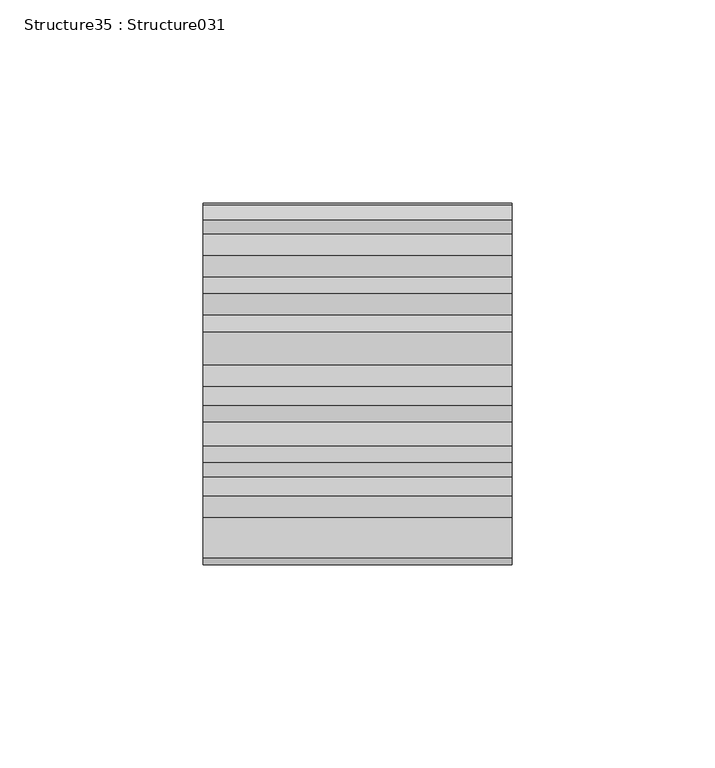
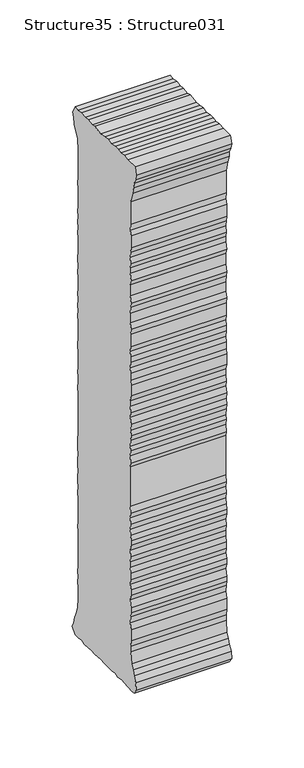
"""IFC4 building model written with IfcOpenShell, lengths in millimetres: proxy geometry, Structure35 : Structure031."""

from ifc_helpers import new_model, si_unit, frame, origin, place, context, project, spatial, polyline, outline, extrude, source, transform, mapped, element, save


def structure35_structure031_ddc4721e(model_context):
    return source(origin(), model_context, "Body", "SweptSolid", [
        extrude(outline(polyline([(252419.4433888, 3575.6853037), (252421.1924077, 3569.8268927), (252423.5431533, 3565.1254015), (252424.7113053, 3559.8671125), (252427.0604463, 3555.1848766), (252422.9606818, 3550.4833855), (252418.8609173, 3550.4833855), (252413.5769547, 3551.6675836), (252410.0580571, 3550.4833855), (252404.7917451, 3550.4833855), (252400.1095092, 3551.0658569), (252396.0097447, 3550.4833855), (252391.3162766, 3551.0658569), (252387.2068845, 3551.6675836), (252382.5326716, 3551.0658569), (252371.974374, 3551.0658569), (252367.2985565, 3551.6675836), (252363.7812634, 3550.4833855), (252358.5053238, 3551.6675836), (252354.9864262, 3551.0658569), (252349.1296198, 3551.0658569), (252344.4457793, 3550.4833855), (252340.9284862, 3551.0658569), (252337.9936646, 3555.1848766), (252338.5777406, 3561.025637), (252340.9284862, 3565.7094775), (252342.6871327, 3569.8268927), (252344.4457793, 3573.9266571), (252345.6107221, 3583.2863152), (252345.6107221, 3587.9685511), (252345.0378783, 3592.6700423), (252345.0378783, 3602.0280957), (252346.1947982, 3607.3393366), (252345.6107221, 3612.5976255), (252345.0378783, 3616.69739), (252345.0378783, 3620.7971545), (252346.1947982, 3626.6571701), (252345.0378783, 3631.3410106), (252345.0378783, 3636.0408972), (252346.1947982, 3640.114988), (252345.6107221, 3644.2420307), (252345.6107221, 3649.5003197), (252346.1947982, 3654.1841602), (252346.1947982, 3658.8840468), (252345.6107221, 3663.5598643), (252346.1947982, 3668.8261762), (252345.0378783, 3673.5276674), (252345.0378783, 3677.6274319), (252345.6107221, 3681.7271964), (252346.1947982, 3686.4030139), (252345.6107221, 3691.0868544), (252346.1947982, 3696.3884676), (252345.6107221, 3700.4705815), (252346.1947982, 3705.7545441), (252346.1947982, 3739.1592005), (252345.6107221, 3742.6748889), (252346.1947982, 3748.5429276), (252345.6107221, 3753.2171405), (252346.1947982, 3756.7440611), (252345.6107221, 3762.0023501), (252345.0378783, 3766.1021146), (252345.6107221, 3770.8036057), (252345.0378783, 3776.0618947), (252346.1947982, 3781.3282066), (252345.6107221, 3785.4456218), (252346.1947982, 3790.7039107), (252346.1947982, 3795.4037973), (252345.0378783, 3800.0876378), (252345.0378783, 3808.8888934), (252345.6107221, 3812.9726119), (252345.6107221, 3818.8310229), (252346.1947982, 3822.932392), (252345.6107221, 3828.2163546), (252345.6107221, 3832.8921721), (252346.1947982, 3836.9919366), (252345.6107221, 3841.0900965), (252345.6107221, 3851.6612309), (252345.0378783, 3856.3161885), (252346.1947982, 3861.0192843), (252346.1947982, 3869.2444869), (252345.6107221, 3874.5043805), (252345.0378783, 3878.5784713), (252346.1947982, 3883.8881076), (252346.1947982, 3893.246161), (252345.0378783, 3897.3475301), (252346.1947982, 3903.2059411), (252346.1947982, 3907.888177), (252345.6107221, 3911.4054701), (252346.1947982, 3916.6653636), (252345.6107221, 3921.3748778), (252345.0378783, 3925.4746423), (252345.0378783, 3935.4328178), (252346.1947982, 3939.5325823), (252345.6107221, 3944.8165449), (252345.6107221, 3964.1343784), (252343.2712088, 3972.3627903), (252341.5189807, 3978.2035506), (252340.9284862, 3982.3225704), (252339.1698397, 3986.4046842), (252337.9936646, 3991.0788971), (252339.7539157, 3996.9645864), (252349.7120912, 3996.9645864), (252354.9864262, 3997.5486624), (252359.6798943, 3996.9645864), (252363.1971874, 3997.5486624), (252367.2985565, 3997.5486624), (252373.1569675, 3996.390138), (252377.2583366, 3997.5486624), (252381.9405725, 3996.9645864), (252387.2068845, 3996.390138), (252395.4160411, 3997.5486624), (252399.5174101, 3996.390138), (252404.7917451, 3997.5486624), (252408.9011372, 3996.9645864), (252414.1674492, 3997.5486624), (252419.4433888, 3996.390138), (252422.9606818, 3997.5486624), (252426.4795795, 3991.0788971), (252424.7113053, 3987.5792547), (252424.1272293, 3981.7208437), (252419.4433888, 3972.3627903), (252418.8609173, 3962.9774586), (252418.8609173, 3940.718385), (252419.4433888, 3935.4328178), (252418.2688183, 3931.3346579), (252418.2688183, 3916.0909152), (252419.4433888, 3911.4054701), (252418.8609173, 3906.7328618), (252419.4433888, 3902.6314927), (252418.8609173, 3897.3475301), (252419.4433888, 3893.246161), (252418.8609173, 3888.5623205), (252418.2688183, 3884.4609514), (252418.2688183, 3879.7610648), (252419.4433888, 3870.4030114), (252418.8609173, 3865.1190488), (252419.4433888, 3859.8591552), (252418.2688183, 3855.7353217), (252418.2688183, 3845.8012153), (252419.4433888, 3842.2758992), (252418.8609173, 3836.4174882), (252419.4433888, 3831.732043), (252418.2688183, 3827.6162325), (252419.4433888, 3822.932392), (252418.8609173, 3817.6741031), (252418.8609173, 3813.5743386), (252418.2688183, 3808.8888934), (252418.2688183, 3804.1890069), (252419.4433888, 3798.9050443), (252418.2688183, 3790.7039107), (252418.2688183, 3780.1616592), (252419.4433888, 3775.4874463), (252418.8609173, 3771.9605256), (252418.2688183, 3767.2590344), (252419.4433888, 3762.5848215), (252418.8609173, 3756.7440611), (252418.2688183, 3752.04257), (252418.2688183, 3747.3587295), (252418.8609173, 3742.6748889), (252418.2688183, 3737.9750024), (252418.2688183, 3733.2991849), (252418.8609173, 3728.5992983), (252418.2688183, 3723.9154578), (252419.4433888, 3719.2316172), (252419.4433888, 3711.0304837), (252418.8609173, 3705.7545441), (252419.4433888, 3701.6547796), (252419.4433888, 3696.3884676), (252418.2688183, 3692.2710525), (252419.4433888, 3687.0127636), (252419.4433888, 3682.3289231), (252418.8609173, 3678.2018803), (252419.4433888, 3673.5276674), (252418.2688183, 3668.2437048), (252418.8609173, 3664.1423357), (252418.2688183, 3659.4584952), (252418.8609173, 3654.7842823), (252418.8609173, 3648.9258713), (252419.4433888, 3644.8245022), (252418.8609173, 3640.114988), (252418.8609173, 3634.856699), (252418.2688183, 3631.3410106), (252418.2688183, 3620.7971545), (252418.8609173, 3617.2718384), (252418.8609173, 3611.4134274), (252419.4433888, 3606.7295868), (252418.8609173, 3602.0280957), (252419.4433888, 3598.5284533), (252418.8609173, 3592.6700423), (252418.8609173, 3583.8864372), (252419.4433888, 3575.6853037)])), frame((-38594.2176606, 0.0, 0.0), z_axis=(1.0, 0.0, 0.0), x_axis=(0.0, 1.0, 0.0)), (0.0, 0.0, 1.0), 76.2),
    ])


if __name__ == "__main__":
    model = new_model("IFC4")
    model_context = context("Model", 3, world=origin())
    ifc_project = project(units=[si_unit("LENGTHUNIT", "METRE", prefix="MILLI")], contexts=[model_context])
    site = spatial("IfcSite", under=ifc_project)
    building = spatial("IfcBuilding", under=site)
    placement = place(None, origin())
    structure35_structure031_shape = structure35_structure031_ddc4721e(model_context)
    element("IfcBuildingElementProxy", 1, Name="Structure35 : Structure031", ObjectType="Structure35 : Structure031", at=placement, inside=building, context=model_context, shape_type="MappedRepresentation", body=[
        mapped(structure35_structure031_shape, transform((0.0, 0.0, 0.0), x_axis=(1.0, 0.0, 0.0), y_axis=(0.0, 1.0, 0.0), z_axis=(0.0, 0.0, 1.0))),
    ])
    save(model, "model.ifc")

# Revit data of these elements
# Type "Structure35 : Structure031"
#   NameOverride = "Structure031"
# Element 1 (IfcBuildingElementProxy, "Structure35 : Structure031")
#   Materials on its faces: "BRUSHED ALUM. LETTERING"
# Materials
#   "BRUSHED ALUM. LETTERING": class "Unassigned", colour RGB 169 181 186, transparency 0, Cost = 0
